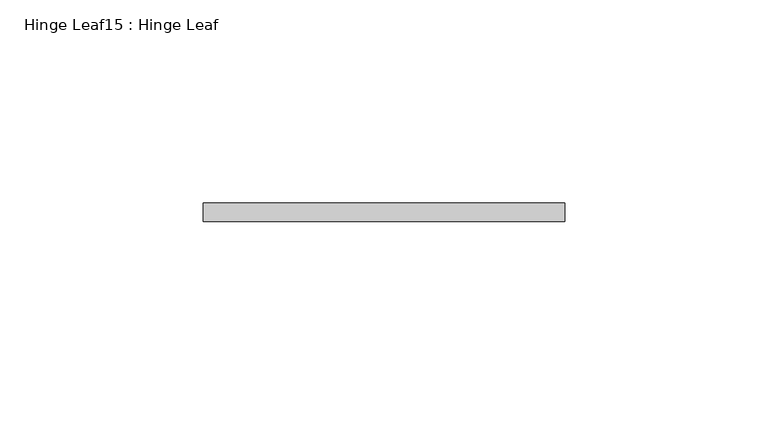
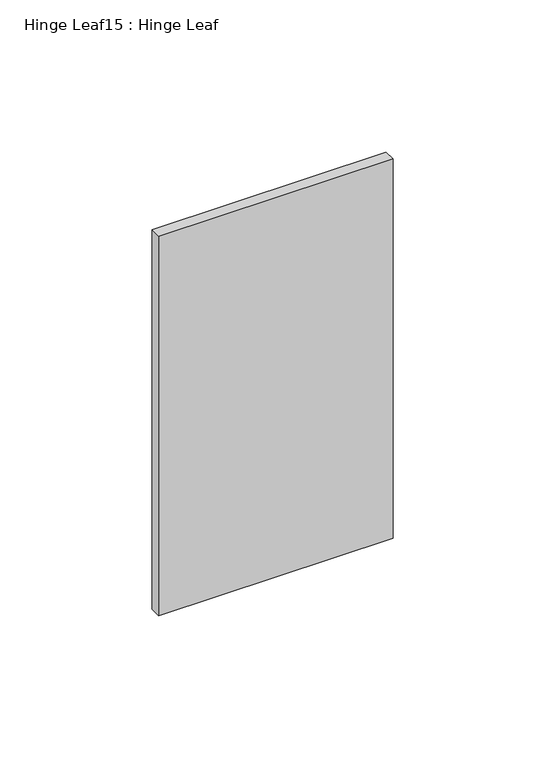
"""IFC4 building model written with IfcOpenShell, lengths in millimetres: proxy geometry, Hinge Leaf15 : Hinge Leaf."""

import ifcopenshell
import ifcopenshell.guid

model = None  # the IFC model being written
_history = None  # IfcOwnerHistory: only IFC2X3 demands one
_inside = {}  # id of a spatial element -> (the spatial element, [elements in it])
_under = {}  # id of a project, library or spatial element -> (it, [spatial elements below it])
_declared = {}  # id of a project -> (the project, [libraries it declares])
_typed = {}  # id of a type object -> (the type object, [elements of that type])
_made_of = {}  # id of a material, layer set ... -> (it, [elements and type objects made of it])


def new_model(schema):
    """Start an empty IFC model of exactly this schema.

    Asked for "IFC4X3", IfcOpenShell would pick the latest addendum, in which some entities
    have other attributes; the version numbers below select the first issue.
    IFC2X3 requires an IfcOwnerHistory on every rooted entity: one is made here for all.
    """
    global model, _history
    if schema == "IFC4X3":
        model = ifcopenshell.file(schema_version=(4, 3, 0, 0))
    else:
        model = ifcopenshell.file(schema=schema)
    _inside.clear()
    _under.clear()
    _declared.clear()
    _typed.clear()
    _made_of.clear()
    _history = None
    if model.schema == "IFC2X3":
        org = make("IfcOrganization", Name="unknown")
        user = make(
            "IfcPersonAndOrganization",
            ThePerson=make("IfcPerson", FamilyName="unknown"),
            TheOrganization=org,
        )
        app = make(
            "IfcApplication",
            ApplicationDeveloper=org,
            Version="unknown",
            ApplicationFullName="unknown",
            ApplicationIdentifier="unknown",
        )
        _history = make(
            "IfcOwnerHistory",
            OwningUser=user,
            OwningApplication=app,
            ChangeAction="ADDED",
            CreationDate=0,
        )
    return model


def make(cls, **values):
    """One entity of the class cls with the attributes given. An attribute that is None is left unset."""
    return model.create_entity(
        cls, **{name: value for name, value in values.items() if value is not None}
    )


def rooted(cls, **values):
    """An entity with a GlobalId (a new one), such as an element, a storey or a relation."""
    return make(cls, GlobalId=ifcopenshell.guid.new(), OwnerHistory=_history, **values)


def si_unit(unit_type, name, prefix=None):
    """IfcSIUnit, for example si_unit("LENGTHUNIT", "METRE", prefix="MILLI")."""
    return make("IfcSIUnit", UnitType=unit_type, Prefix=prefix, Name=name)


def assignment(units):
    """IfcUnitAssignment: the units of a project."""
    return None if units is None else make("IfcUnitAssignment", Units=units)


def point(xyz):
    """IfcCartesianPoint."""
    return None if xyz is None else make("IfcCartesianPoint", Coordinates=xyz)


def direction(xyz):
    """IfcDirection."""
    return None if xyz is None else make("IfcDirection", DirectionRatios=xyz)


def frame(location, z_axis=None, x_axis=None):
    """IfcAxis2Placement3D, a coordinate frame: its origin and axes. An axis left out is left unset."""
    return make(
        "IfcAxis2Placement3D",
        Location=point(location),
        Axis=direction(z_axis),
        RefDirection=direction(x_axis),
    )


def origin():
    """The frame at (0, 0, 0) with its axes left unset."""
    return frame((0.0, 0.0, 0.0))


def place(relative_to, where):
    """IfcLocalPlacement: puts the frame where relative to a parent placement (None: the world)."""
    return make(
        "IfcLocalPlacement", PlacementRelTo=relative_to, RelativePlacement=where
    )


def context(
    kind, dimensions, precision=None, world=None, true_north=None, identifier=None
):
    """IfcGeometricRepresentationContext, for example the 3D "Model" context."""
    return make(
        "IfcGeometricRepresentationContext",
        ContextIdentifier=identifier,
        ContextType=kind,
        CoordinateSpaceDimension=dimensions,
        Precision=precision,
        WorldCoordinateSystem=world,
        TrueNorth=true_north,
    )


def project(units=None, contexts=None):
    """IfcProject with its units and contexts."""
    return rooted(
        "IfcProject",
        Name="project",
        RepresentationContexts=contexts,
        UnitsInContext=assignment(units),
    )


def spatial(cls, under=None, at=None, **own):
    """A site, building, storey or space (cls), placed at a placement, below another one or the project."""
    s = rooted(cls, ObjectPlacement=at, **own)
    if under is not None:
        _under.setdefault(under.id(), (under, []))[1].append(s)
    return s


def polyline(points):
    """IfcPolyline through the points."""
    return make("IfcPolyline", Points=[point(p) for p in points])


def outline(outer, holes=None, kind="AREA"):
    """IfcArbitraryClosedProfileDef: a profile drawn as a closed curve; with holes, ...WithVoids."""
    if holes is None:
        return make("IfcArbitraryClosedProfileDef", ProfileType=kind, OuterCurve=outer)
    return make(
        "IfcArbitraryProfileDefWithVoids",
        ProfileType=kind,
        OuterCurve=outer,
        InnerCurves=holes,
    )


def extrude(swept, where, along, depth):
    """IfcExtrudedAreaSolid: the profile swept, set in the frame where, extruded along a direction by depth."""
    return make(
        "IfcExtrudedAreaSolid",
        SweptArea=swept,
        Position=where,
        ExtrudedDirection=direction(along),
        Depth=depth,
    )


def shape(context_of_items, identifier, shape_type, items):
    """IfcShapeRepresentation: the items that make up one representation, for example the "Body"."""
    return make(
        "IfcShapeRepresentation",
        ContextOfItems=context_of_items,
        RepresentationIdentifier=identifier,
        RepresentationType=shape_type,
        Items=items,
    )


def source(mapping_origin, context_of_items, identifier, shape_type, items):
    """IfcRepresentationMap: a shape defined once, which mapped items show again and again."""
    return make(
        "IfcRepresentationMap",
        MappingOrigin=mapping_origin,
        MappedRepresentation=shape(context_of_items, identifier, shape_type, items),
    )


def transform(
    local_origin,
    x_axis=None,
    y_axis=None,
    z_axis=None,
    scale=None,
    scale2=None,
    scale3=None,
    uniform=True,
):
    """IfcCartesianTransformationOperator3D, or its non-uniform kind. x_axis, y_axis, z_axis: its Axis1, 2, 3."""
    if uniform:
        return make(
            "IfcCartesianTransformationOperator3D",
            Axis1=direction(x_axis),
            Axis2=direction(y_axis),
            LocalOrigin=point(local_origin),
            Scale=scale,
            Axis3=direction(z_axis),
        )
    return make(
        "IfcCartesianTransformationOperator3DnonUniform",
        Axis1=direction(x_axis),
        Axis2=direction(y_axis),
        LocalOrigin=point(local_origin),
        Scale=scale,
        Axis3=direction(z_axis),
        Scale2=scale2,
        Scale3=scale3,
    )


def mapped(mapping_source, mapping_target):
    """IfcMappedItem: shows the shape of a source again, moved by a transform."""
    return make(
        "IfcMappedItem", MappingSource=mapping_source, MappingTarget=mapping_target
    )


def made_of(thing, what):
    """Note that an element or type object is made of a material, layer set ...; save() writes the relation."""
    if what is not None:
        _made_of.setdefault(what.id(), (what, []))[1].append(thing)
    return thing


def element(
    cls,
    number,
    at=None,
    inside=None,
    cuts=None,
    type_object=None,
    material=None,
    context=None,
    identifier="Body",
    shape_type=None,
    held_by="IfcProductDefinitionShape",
    body=None,
    shapes=None,
    **own,
):
    """One element of the class cls, such as IfcWall. Its Tag is "e" and its number.

    at: its placement. inside: the storey or other place that contains it. cuts: it is an
    opening in that element (IfcRelVoidsElement). A single representation is given by context,
    identifier, shape_type and body (its items); several are given by shapes. held_by: the class
    of the entity that holds the representations. save() writes the other relations.
    """
    e = rooted(cls, Tag="e%d" % number, ObjectPlacement=at, **own)
    if body is not None:
        shapes = [shape(context, identifier, shape_type, body)]
    if shapes is not None:
        e.Representation = make(held_by, Representations=shapes)
    if inside is not None:
        _inside.setdefault(inside.id(), (inside, []))[1].append(e)
    if cuts is not None:
        rooted(
            "IfcRelVoidsElement", RelatingBuildingElement=cuts, RelatedOpeningElement=e
        )
    if type_object is not None:
        _typed.setdefault(type_object.id(), (type_object, []))[1].append(e)
    return made_of(e, material)


def aggregate(whole, parts):
    """IfcRelAggregates: a whole, such as a stair, and the parts it consists of."""
    return rooted("IfcRelAggregates", RelatingObject=whole, RelatedObjects=parts)


def save(model, path):
    """Write the relations noted so far, then the file.

    IfcRelAggregates (storeys below a building ...), IfcRelContainedInSpatialStructure (elements
    in a storey), IfcRelDefinesByType, IfcRelAssociatesMaterial and IfcRelDeclares: one each for
    every whole, place, type object, material and project.
    """
    for whole, parts in _under.values():
        aggregate(whole, parts)
    for where, things in _inside.values():
        rooted(
            "IfcRelContainedInSpatialStructure",
            RelatedElements=things,
            RelatingStructure=where,
        )
    for kind, things in _typed.values():
        rooted("IfcRelDefinesByType", RelatedObjects=things, RelatingType=kind)
    for what, things in _made_of.values():
        rooted("IfcRelAssociatesMaterial", RelatedObjects=things, RelatingMaterial=what)
    for by, libraries in _declared.values():
        rooted("IfcRelDeclares", RelatingContext=by, RelatedDefinitions=libraries)
    model.write(path)


def hinge_leaf15_hinge_leaf_b84fefac(model_context):
    return source(origin(), model_context, "Body", "SweptSolid", [
        extrude(outline(polyline([(587327.7934739, -534096.6663841), (587416.6934739, -534096.6663841), (587416.6934739, -534101.2383841), (587327.7934739, -534101.2383841), (587327.7934739, -534096.6663841)])), frame((0.0, 0.0, 311.15), z_axis=(0.0, 0.0, 1.0), x_axis=(1.0, 0.0, 0.0)), (0.0, 0.0, 1.0), 152.4),
    ])


if __name__ == "__main__":
    model = new_model("IFC4")
    model_context = context("Model", 3, world=origin())
    ifc_project = project(units=[si_unit("LENGTHUNIT", "METRE", prefix="MILLI")], contexts=[model_context])
    site = spatial("IfcSite", under=ifc_project)
    building = spatial("IfcBuilding", under=site)
    placement = place(None, origin())
    hinge_leaf15_hinge_leaf_shape = hinge_leaf15_hinge_leaf_b84fefac(model_context)
    element("IfcBuildingElementProxy", 1, Name="Hinge Leaf15 : Hinge Leaf", ObjectType="Hinge Leaf15 : Hinge Leaf", at=placement, inside=building, context=model_context, shape_type="MappedRepresentation", body=[
        mapped(hinge_leaf15_hinge_leaf_shape, transform((0.0, 0.0, 0.0), x_axis=(1.0, 0.0, 0.0), y_axis=(0.0, 1.0, 0.0), z_axis=(0.0, 0.0, 1.0))),
    ])
    save(model, "model.ifc")

# Revit data of these elements
# Element 1 (IfcBuildingElementProxy, "Hinge Leaf15 : Hinge Leaf")
#   Materials on its faces: "6\"X6\" WELD-ON STL BUTT HINGE"
# Materials
#   "6\"X6\" WELD-ON STL BUTT HINGE": class "Metal", colour RGB 189 187 185, transparency 0, Description = "Carbon steel", Cost = 0
